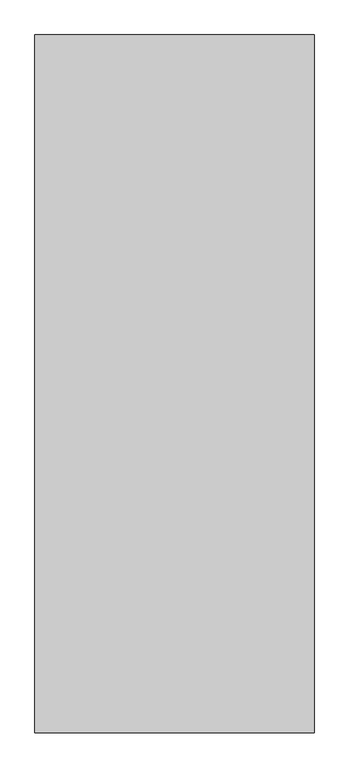
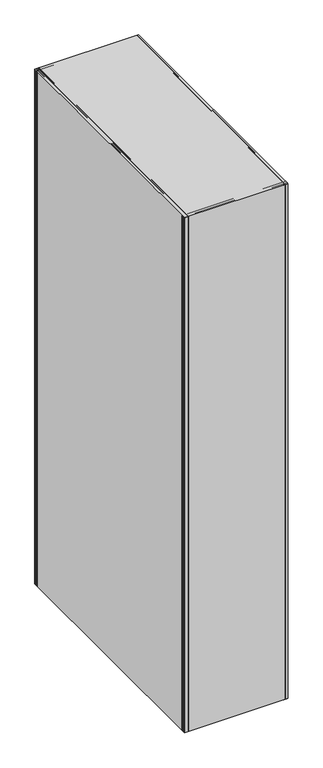
"""IFC4 building model written with IfcOpenShell, lengths in millimetres: beam geometry, LF02ZBK001_DIKE WALL_RC : Dike_Thk.400_EW2."""

from ifc_helpers import new_model, si_unit, origin, origin_with_axes, place, context, project, spatial, polyline, outline, extrude, source, transform, mapped, element, save


def beam_97304d78(model_context):
    return source(origin(), model_context, "Body", "SweptSolid", [
        extrude(outline(polyline([(200.0, -500.0), (-200.0, -500.0), (-200.0, 500.0), (200.0, 500.0), (200.0, -500.0)])), origin_with_axes(), (0.0, 0.0, 1.0), 2100.0),
        extrude(outline(polyline([(-200.0, -485.0), (-200.0, -484.0), (200.0, -484.0), (200.0, -485.0), (-200.0, -485.0)])), origin_with_axes(), (0.0, 0.0, 1.0), 2100.0),
        extrude(outline(polyline([(-200.0, -490.0), (-200.0, -489.0), (200.0, -489.0), (200.0, -490.0), (-200.0, -490.0)])), origin_with_axes(), (0.0, 0.0, 1.0), 2100.0),
        extrude(outline(polyline([(-200.0, -495.0), (-200.0, -494.0), (200.0, -494.0), (200.0, -495.0), (-200.0, -495.0)])), origin_with_axes(), (0.0, 0.0, 1.0), 2100.0),
        extrude(outline(polyline([(-200.0, 485.0), (200.0, 485.0), (200.0, 484.0), (-200.0, 484.0), (-200.0, 485.0)])), origin_with_axes(), (0.0, 0.0, 1.0), 2100.0),
        extrude(outline(polyline([(-200.0, 490.0), (200.0, 490.0), (200.0, 489.0), (-200.0, 489.0), (-200.0, 490.0)])), origin_with_axes(), (0.0, 0.0, 1.0), 2100.0),
        extrude(outline(polyline([(-200.0, 495.0), (200.0, 495.0), (200.0, 494.0), (-200.0, 494.0), (-200.0, 495.0)])), origin_with_axes(), (0.0, 0.0, 1.0), 2100.0),
        extrude(outline(polyline([(184.0, 500.0), (185.0, 500.0), (185.0, -500.0), (184.0, -500.0), (184.0, 500.0)])), origin_with_axes(), (0.0, 0.0, 1.0), 2100.0),
        extrude(outline(polyline([(189.0, 500.0), (190.0, 500.0), (190.0, -500.0), (189.0, -500.0), (189.0, 500.0)])), origin_with_axes(), (0.0, 0.0, 1.0), 2100.0),
        extrude(outline(polyline([(194.0, 500.0), (195.0, 500.0), (195.0, -500.0), (194.0, -500.0), (194.0, 500.0)])), origin_with_axes(), (0.0, 0.0, 1.0), 2100.0),
        extrude(outline(polyline([(-184.0, 500.0), (-184.0, -500.0), (-185.0, -500.0), (-185.0, 500.0), (-184.0, 500.0)])), origin_with_axes(), (0.0, 0.0, 1.0), 2100.0),
        extrude(outline(polyline([(-189.0, 500.0), (-189.0, -500.0), (-190.0, -500.0), (-190.0, 500.0), (-189.0, 500.0)])), origin_with_axes(), (0.0, 0.0, 1.0), 2100.0),
        extrude(outline(polyline([(-194.0, 500.0), (-194.0, -500.0), (-195.0, -500.0), (-195.0, 500.0), (-194.0, 500.0)])), origin_with_axes(), (0.0, 0.0, 1.0), 2100.0),
    ])


if __name__ == "__main__":
    model = new_model("IFC4")
    model_context = context("Model", 3, world=origin())
    ifc_project = project(units=[si_unit("LENGTHUNIT", "METRE", prefix="MILLI")], contexts=[model_context])
    site = spatial("IfcSite", under=ifc_project)
    building = spatial("IfcBuilding", under=site)
    placement = place(None, origin())
    beam_shape = beam_97304d78(model_context)
    element("IfcBeam", 1, ObjectType="LF02ZBK001_DIKE WALL_RC : Dike_Thk.400_EW2", at=placement, inside=building, context=model_context, shape_type="MappedRepresentation", body=[
        mapped(beam_shape, transform((0.0, 0.0, 0.0), x_axis=(1.0, 0.0, 0.0), y_axis=(0.0, 1.0, 0.0), z_axis=(0.0, 0.0, 1.0))),
    ])
    save(model, "model.ifc")

# Revit data of these elements
# Type "LF02ZBK001_DIKE WALL_RC : Dike_Thk.400_EW2"
#   Dike_thk = 400 mm
#   Dike_Length [instance default] = 3000 mm
#   Dike_Hight = 2100 mm
#   c2_visible = yes
#   c3_material [instance default] = none
#   c2_material 3 [instance default] = none
#   c2_material 2 [instance default] = none
#   c2_material 1 [instance default] = none
#   c1_material [instance default] = none
#   Default Elevation = 0
# Element 1 (IfcBeam, "LF02ZBK001_DIKE WALL_RC : Dike_Thk.400_EW2")
#   Dike_Length = 1000 mm
